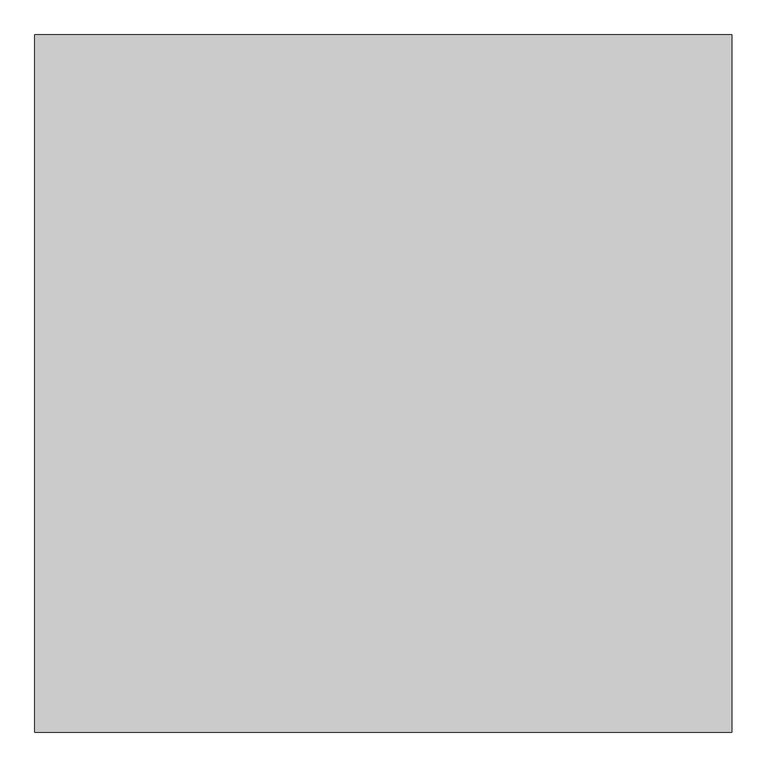
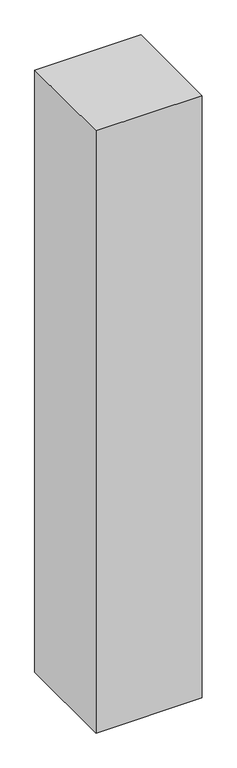
"""IFC4 building model written with IfcOpenShell, lengths in millimetres: proxy geometry, Space Planning Box_hec : Space Planning Box_hec."""

from ifc_helpers import new_model, si_unit, origin, origin_with_axes, place, context, project, spatial, polyline, outline, extrude, source, transform, mapped, element, save


def generic_models_ed4b717c(model_context):
    return source(origin(), model_context, "Body", "SweptSolid", [
        extrude(outline(polyline([(500.0, 500.0), (500.0, -500.0), (-500.0, -500.0), (-500.0, 500.0), (500.0, 500.0)])), origin_with_axes(), (0.0, 0.0, 1.0), 6000.0),
    ])


if __name__ == "__main__":
    model = new_model("IFC4")
    model_context = context("Model", 3, world=origin())
    ifc_project = project(units=[si_unit("LENGTHUNIT", "METRE", prefix="MILLI")], contexts=[model_context])
    site = spatial("IfcSite", under=ifc_project)
    building = spatial("IfcBuilding", under=site)
    placement = place(None, origin())
    generic_models_shape = generic_models_ed4b717c(model_context)
    element("IfcBuildingElementProxy", 1, Name="Space Planning Box_hec : Space Planning Box_hec", ObjectType="Space Planning Box_hec : Space Planning Box_hec", at=placement, inside=building, context=model_context, shape_type="MappedRepresentation", body=[
        mapped(generic_models_shape, transform((0.0, 0.0, 0.0), x_axis=(1.0, 0.0, 0.0), y_axis=(0.0, 1.0, 0.0), z_axis=(0.0, 0.0, 1.0))),
    ])
    save(model, "model.ifc")

# Revit data of these elements
# Type "Space Planning Box_hec : Space Planning Box_hec"
#   Type Comments = "..."
#   Room Name [instance default] = "?"
#   Interior Finish [instance default] = ""
#   Exterior Finish [instance default] = ""
#   Department [instance default] = ""
#   Assembly Code = "..."
#   Width [instance default] = 1524 mm
#   Program Area [instance default] = 0.00 m²
#   Length [instance default] = 1524 mm
#   Height [instance default] = 1524 mm
#   Area [instance default] = 2.32258 m²
#   Fill Color [instance default] = Cyan
#   Default Elevation = 0
# Element 1 (IfcBuildingElementProxy, "Space Planning Box_hec : Space Planning Box_hec")
#   Room Name = "Fire Gas Room"
#   Interior Finish = "IF1"
#   Exterior Finish = "EF1"
#   Department = "SF"
#   Width = 1000 mm
#   Length = 1000 mm
#   Height = 6000 mm
#   Area = 1.00 m²
#   Materials on its faces: "Cyan"
# Materials
#   "Cyan": class "Generic", colour RGB 0 255 255, transparency 0.2, Cost = 0
